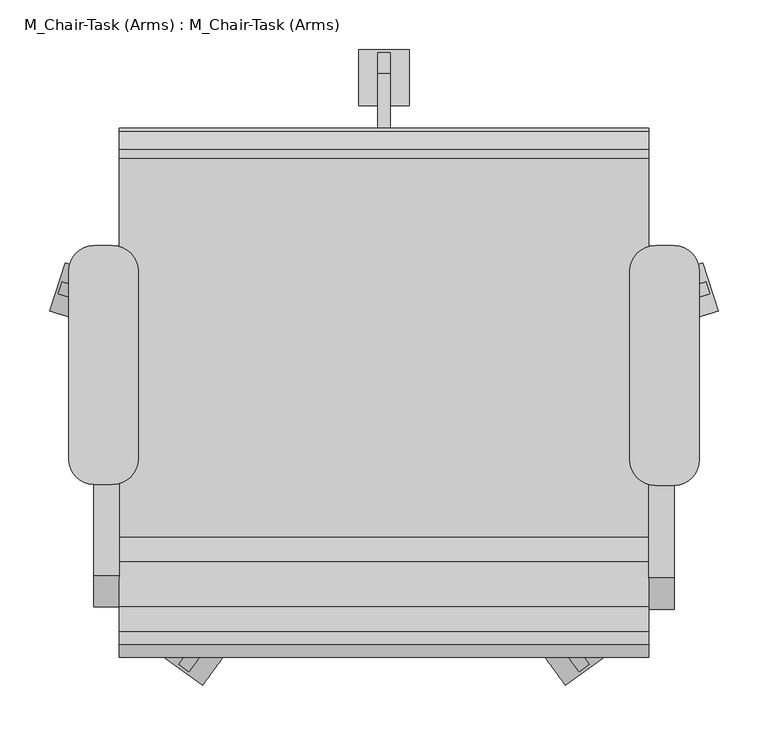
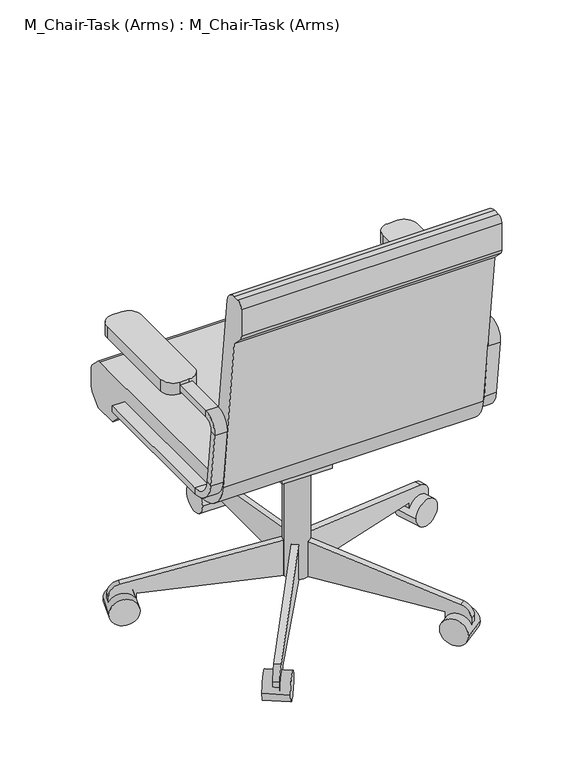
"""IFC4 building model written with IfcOpenShell, lengths in millimetres: furniture geometry, M_Chair-Task (Arms) : M_Chair-Task (Arms)."""

from ifc_helpers import new_model, si_unit, point, frame, frame_2d, origin, place, context, project, spatial, polyline, circle_curve, trimmed, segment, composite_curve, outline, extrude, source, transform, mapped, element, save
from ifc_brep_helpers import plane_surface, cylinder_surface, revolved_surface, advanced_brep


def m_chair_task_arms_m_chair_task_arms_fa5a08ef(model_context):
    return source(origin(), model_context, "Body", "SolidModel", [
        extrude(outline(composite_curve([segment(polyline([(433.0908197, -74.2028048), (414.0408197, -74.2028048)]), True, "CONTINUOUS"), segment(trimmed(circle_curve(frame_2d((414.0408197, -48.8028048)), 25.4), [point((414.0408197, -74.2028048))], [point((388.6408197, -48.8028048))], False, "CARTESIAN"), True, "CONTINUOUS"), segment(polyline([(388.6408197, -48.8028048), (388.6408197, 141.6319091)]), True, "CONTINUOUS"), segment(trimmed(circle_curve(frame_2d((414.0408197, 141.6319091)), 25.4), [point((388.6408197, 141.6319091))], [point((414.0408197, 167.0319091))], False, "CARTESIAN"), True, "CONTINUOUS"), segment(polyline([(414.0408197, 167.0319091), (433.0908197, 167.0319091)]), True, "CONTINUOUS"), segment(trimmed(circle_curve(frame_2d((433.0908197, 141.6319091)), 25.4), [point((433.0908197, 167.0319091))], [point((458.4908197, 141.6319091))], False, "CARTESIAN"), True, "CONTINUOUS"), segment(polyline([(458.4908197, 141.6319091), (458.4908197, -48.8028048)]), True, "CONTINUOUS"), segment(trimmed(circle_curve(frame_2d((433.0908197, -48.8028048)), 25.4), [point((458.4908197, -48.8028048))], [point((433.0908197, -74.2028048))], False, "CARTESIAN"), True, "CONTINUOUS")], self_intersect=False)), frame((0.0, 0.0, 596.9), z_axis=(0.0, 0.0, 1.0), x_axis=(1.0, 0.0, 0.0)), (0.0, 0.0, 1.0), 25.4),
        extrude(outline(composite_curve([segment(polyline([(-132.0591803, -73.1575984), (-151.1091803, -73.1575984)]), True, "CONTINUOUS"), segment(trimmed(circle_curve(frame_2d((-151.1091803, -47.7575984)), 25.4), [point((-151.1091803, -73.1575984))], [point((-176.5091803, -47.7575984))], False, "CARTESIAN"), True, "CONTINUOUS"), segment(polyline([(-176.5091803, -47.7575984), (-176.5091803, 141.6319091)]), True, "CONTINUOUS"), segment(trimmed(circle_curve(frame_2d((-151.1091803, 141.6319091)), 25.4), [point((-176.5091803, 141.6319091))], [point((-151.1091803, 167.0319091))], False, "CARTESIAN"), True, "CONTINUOUS"), segment(polyline([(-151.1091803, 167.0319091), (-132.0591803, 167.0319091)]), True, "CONTINUOUS"), segment(trimmed(circle_curve(frame_2d((-132.0591803, 141.6319091)), 25.4), [point((-132.0591803, 167.0319091))], [point((-106.6591803, 141.6319091))], False, "CARTESIAN"), True, "CONTINUOUS"), segment(polyline([(-106.6591803, 141.6319091), (-106.6591803, -47.7575984)]), True, "CONTINUOUS"), segment(trimmed(circle_curve(frame_2d((-132.0591803, -47.7575984)), 25.4), [point((-106.6591803, -47.7575984))], [point((-132.0591803, -73.1575984))], False, "CARTESIAN"), True, "CONTINUOUS")], self_intersect=False)), frame((0.0, 0.0, 596.9), z_axis=(0.0, 0.0, 1.0), x_axis=(1.0, 0.0, 0.0)), (0.0, 0.0, 1.0), 25.4),
        advanced_brep(
        [(-151.1091803, 167.0319091, 412.75), (-151.1091803, 167.0319091, 425.45), (-125.7091803, 167.0319091, 425.45), (-125.7091803, 167.0319091, 412.75), (-151.1091803, -126.2388651, 412.75), (-151.1091803, -126.2388651, 425.45), (-125.7091803, -126.2388651, 425.45), (-125.7091803, -126.2388651, 412.75), (-151.1091803, -170.3844094, 464.7064065), (-151.1091803, -182.9974221, 463.2225227), (-125.7091803, -170.3844094, 464.7064065), (-125.7091803, -182.9974221, 463.2225227), (-151.1091803, -196.7936301, 580.4902904), (-151.1091803, -184.1806174, 581.9741742), (-125.7091803, -184.1806174, 581.9741742), (-125.7091803, -196.7936301, 580.4902904), (-151.1091803, -165.2610984, 603.25), (-151.1091803, -165.2610984, 615.95), (-125.7091803, -165.2610984, 603.25), (-125.7091803, -165.2610984, 615.95), (-151.1091803, 18.9459016, 615.95), (-125.7091803, 18.9459016, 615.95), (-125.7091803, 18.9459016, 603.25), (-151.1091803, 18.9459016, 603.25)],
        [
            (0, 1),
            (1, 2),
            (2, 3),
            (3, 0),
            (0, 4),
            (4, 5),
            (5, 1),
            (5, 6),
            (6, 2),
            (6, 7),
            (7, 3),
            (7, 4),
            (8, 5, circle_curve(frame((-151.1091803, -126.2388651, 469.9), z_axis=(1.0, 0.0, 0.0), x_axis=(0.0, 0.0, -1.0)), 44.45)),
            (4, 9, circle_curve(frame((-151.1091803, -126.2388651, 469.9), z_axis=(-1.0, 0.0, 0.0), x_axis=(0.0, 0.0, -1.0)), 57.15)),
            (9, 8),
            (10, 6, circle_curve(frame((-125.7091803, -126.2388651, 469.9), z_axis=(1.0, 0.0, 0.0), x_axis=(0.0, 0.0, -1.0)), 44.45)),
            (8, 10),
            (11, 7, circle_curve(frame((-125.7091803, -126.2388651, 469.9), z_axis=(1.0, 0.0, 0.0), x_axis=(0.0, 0.0, -1.0)), 57.15)),
            (10, 11),
            (11, 9),
            (9, 12),
            (12, 13),
            (13, 8),
            (13, 14),
            (14, 10),
            (14, 15),
            (15, 11),
            (15, 12),
            (16, 13, circle_curve(frame((-151.1091803, -165.2610984, 584.2), z_axis=(1.0, 0.0, 0.0), x_axis=(0.0, -0.9931506043228768, -0.11684124756739202)), 19.05)),
            (12, 17, circle_curve(frame((-151.1091803, -165.2610984, 584.2), z_axis=(-1.0, 0.0, 0.0), x_axis=(0.0, -0.9931506043228768, -0.11684124756739202)), 31.75)),
            (17, 16),
            (18, 14, circle_curve(frame((-125.7091803, -165.2610984, 584.2), z_axis=(1.0, 0.0, 0.0), x_axis=(0.0, -0.9931506043228768, -0.11684124756739202)), 19.05)),
            (16, 18),
            (19, 15, circle_curve(frame((-125.7091803, -165.2610984, 584.2), z_axis=(1.0, 0.0, 0.0), x_axis=(0.0, -0.9931506043228768, -0.11684124756739202)), 31.75)),
            (18, 19),
            (19, 17),
            (20, 21),
            (21, 22),
            (22, 23),
            (23, 20),
            (17, 20),
            (23, 16),
            (22, 18),
            (21, 19),
        ],
        [
            plane_surface(frame((-152.608212, 167.0319091, 419.1), z_axis=(0.0, 1.0, 0.0), x_axis=(0.0, 0.0, -1.0))),
            plane_surface(frame((-151.1091803, 167.0319091, 412.75), z_axis=(-1.0, 0.0, 0.0), x_axis=(0.0, -1.0, 0.0))),
            plane_surface(frame((-151.1091803, 167.0319091, 425.45), z_axis=(0.0, 0.0, 1.0), x_axis=(0.0, -1.0, 0.0))),
            plane_surface(frame((-125.7091803, 167.0319091, 425.45), z_axis=(1.0, 0.0, 0.0), x_axis=(0.0, -1.0, 0.0))),
            plane_surface(frame((-125.7091803, 167.0319091, 412.75), z_axis=(0.0, 0.0, -1.0), x_axis=(0.0, -1.0, 0.0))),
            plane_surface(frame((-151.1091803, -126.2388651, 469.9), z_axis=(-1.0, 0.0, 0.0), x_axis=(0.0, 0.0, -1.0))),
            revolved_surface(polyline([(-151.1091803, -126.2388651, 425.45), (-125.7091803, -126.2388651, 425.45)]), (-138.4091803, -126.2388651, 469.9), (-1.0, 0.0, 0.0)),
            plane_surface(frame((-125.7091803, -126.2388651, 469.9), z_axis=(1.0, 0.0, 0.0), x_axis=(0.0, 0.0, -1.0))),
            cylinder_surface(frame((-138.4091803, -126.2388651, 469.9), z_axis=(-1.0, 0.0, 0.0), x_axis=(0.0, 0.0, -1.0)), 57.15),
            plane_surface(frame((-151.1091803, -182.9974221, 463.2225227), z_axis=(-1.0, 0.0, 0.0), x_axis=(0.0, -0.1168412475673856, 0.9931506043228776))),
            plane_surface(frame((-151.1091803, -170.3844094, 464.7064065), z_axis=(0.0, 0.9931506043228776, 0.1168412475673856), x_axis=(0.0, -0.1168412475673856, 0.9931506043228776))),
            plane_surface(frame((-125.7091803, -170.3844094, 464.7064065), z_axis=(1.0, 0.0, 0.0), x_axis=(0.0, -0.1168412475673856, 0.9931506043228776))),
            plane_surface(frame((-125.7091803, -182.9974221, 463.2225227), z_axis=(0.0, -0.9931506043228776, -0.1168412475673856), x_axis=(0.0, -0.1168412475673856, 0.9931506043228776))),
            plane_surface(frame((-151.1091803, -165.2610984, 584.2), z_axis=(-1.0, 0.0, 0.0), x_axis=(0.0, -0.9931506043228768, -0.11684124756739202))),
            revolved_surface(polyline([(-151.1091803, -184.1806174123508, 581.9741742338413), (-125.7091803, -184.1806174123508, 581.9741742338413)]), (-138.4091803, -165.2610984, 584.2), (-1.0, 0.0, 0.0)),
            plane_surface(frame((-125.7091803, -165.2610984, 584.2), z_axis=(1.0, 0.0, 0.0), x_axis=(0.0, -0.9931506043228768, -0.11684124756739202))),
            cylinder_surface(frame((-138.4091803, -165.2610984, 584.2), z_axis=(-1.0, 0.0, 0.0), x_axis=(0.0, -0.9931506043228768, -0.11684124756739202)), 31.75),
            plane_surface(frame((-152.608212, 18.9459016, 609.6), z_axis=(0.0, 1.0, 0.0), x_axis=(0.0, 0.0, 1.0))),
            plane_surface(frame((-151.1091803, -165.2610984, 615.95), z_axis=(-1.0, 0.0, 0.0), x_axis=(0.0, 1.0, 0.0))),
            plane_surface(frame((-151.1091803, -165.2610984, 603.25), z_axis=(0.0, 0.0, -1.0), x_axis=(0.0, 1.0, 0.0))),
            plane_surface(frame((-125.7091803, -165.2610984, 603.25), z_axis=(1.0, 0.0, 0.0), x_axis=(0.0, 1.0, 0.0))),
            plane_surface(frame((-125.7091803, -165.2610984, 615.95), z_axis=(0.0, 0.0, 1.0), x_axis=(0.0, 1.0, 0.0))),
        ],
        [
            (0, [[1, 2, 3, 4]]),
            (1, [[-1, 5, 6, 7]]),
            (2, [[-2, -7, 8, 9]]),
            (3, [[-3, -9, 10, 11]]),
            (4, [[-4, -11, 12, -5]]),
            (5, [[13, -6, 14, 15]]),
            (6, [[16, -8, -13, 17]]),
            (7, [[18, -10, -16, 19]]),
            (8, [[-14, -12, -18, 20]]),
            (9, [[-15, 21, 22, 23]]),
            (10, [[-17, -23, 24, 25]]),
            (11, [[-19, -25, 26, 27]]),
            (12, [[-20, -27, 28, -21]]),
            (13, [[29, -22, 30, 31]]),
            (14, [[32, -24, -29, 33]]),
            (15, [[34, -26, -32, 35]]),
            (16, [[-30, -28, -34, 36]]),
            (17, [[37, 38, 39, 40]]),
            (18, [[-31, 41, -40, 42]]),
            (19, [[-33, -42, -39, 43]]),
            (20, [[-35, -43, -38, 44]]),
            (21, [[-36, -44, -37, -41]]),
        ],
    ),
        advanced_brep(
        [(433.0908197, 167.0319091, 425.45), (433.0908197, 167.0319091, 412.75), (407.6908197, 167.0319091, 412.75), (407.6908197, 167.0319091, 425.45), (433.0908197, -128.329278, 425.45), (433.0908197, -128.329278, 412.75), (407.6908197, -128.329278, 412.75), (407.6908197, -128.329278, 425.45), (433.0908197, -185.0878351, 463.2225227), (433.0908197, -172.4748224, 464.7064065), (407.6908197, -185.0878351, 463.2225227), (407.6908197, -172.4748224, 464.7064065), (433.0908197, -186.2710303, 581.9741742), (433.0908197, -198.884043, 580.4902904), (407.6908197, -198.884043, 580.4902904), (407.6908197, -186.2710303, 581.9741742), (433.0908197, -167.3515113, 615.95), (433.0908197, -167.3515113, 603.25), (407.6908197, -167.3515113, 615.95), (407.6908197, -167.3515113, 603.25), (433.0908197, 18.9459016, 603.25), (407.6908197, 18.9459016, 603.25), (407.6908197, 18.9459016, 615.95), (433.0908197, 18.9459016, 615.95)],
        [
            (0, 1),
            (1, 2),
            (2, 3),
            (3, 0),
            (0, 4),
            (4, 5),
            (5, 1),
            (5, 6),
            (6, 2),
            (6, 7),
            (7, 3),
            (7, 4),
            (8, 5, circle_curve(frame((433.0908197, -128.329278, 469.9), z_axis=(1.0, 0.0, 0.0), x_axis=(0.0, 0.0, -1.0)), 57.15)),
            (4, 9, circle_curve(frame((433.0908197, -128.329278, 469.9), z_axis=(-1.0, 0.0, 0.0), x_axis=(0.0, 0.0, -1.0)), 44.45)),
            (9, 8),
            (10, 6, circle_curve(frame((407.6908197, -128.329278, 469.9), z_axis=(1.0, 0.0, 0.0), x_axis=(0.0, 0.0, -1.0)), 57.15)),
            (8, 10),
            (11, 7, circle_curve(frame((407.6908197, -128.329278, 469.9), z_axis=(1.0, 0.0, 0.0), x_axis=(0.0, 0.0, -1.0)), 44.45)),
            (10, 11),
            (11, 9),
            (9, 12),
            (12, 13),
            (13, 8),
            (13, 14),
            (14, 10),
            (14, 15),
            (15, 11),
            (15, 12),
            (16, 13, circle_curve(frame((433.0908197, -167.3515113, 584.2), z_axis=(1.0, 0.0, 0.0), x_axis=(0.0, -0.9931506043228767, -0.1168412475673929)), 31.75)),
            (12, 17, circle_curve(frame((433.0908197, -167.3515113, 584.2), z_axis=(-1.0, 0.0, 0.0), x_axis=(0.0, -0.9931506043228767, -0.1168412475673929)), 19.05)),
            (17, 16),
            (18, 14, circle_curve(frame((407.6908197, -167.3515113, 584.2), z_axis=(1.0, 0.0, 0.0), x_axis=(0.0, -0.9931506043228767, -0.1168412475673929)), 31.75)),
            (16, 18),
            (19, 15, circle_curve(frame((407.6908197, -167.3515113, 584.2), z_axis=(1.0, 0.0, 0.0), x_axis=(0.0, -0.9931506043228767, -0.1168412475673929)), 19.05)),
            (18, 19),
            (19, 17),
            (20, 21),
            (21, 22),
            (22, 23),
            (23, 20),
            (17, 20),
            (23, 16),
            (22, 18),
            (21, 19),
        ],
        [
            plane_surface(frame((406.191788, 167.0319091, 419.1), z_axis=(0.0, 1.0, 0.0), x_axis=(0.0, 0.0, -1.0))),
            plane_surface(frame((433.0908197, 167.0319091, 425.45), z_axis=(1.0, 0.0, 0.0), x_axis=(0.0, -1.0, 0.0))),
            plane_surface(frame((433.0908197, 167.0319091, 412.75), z_axis=(0.0, 0.0, -1.0), x_axis=(0.0, -1.0, 0.0))),
            plane_surface(frame((407.6908197, 167.0319091, 412.75), z_axis=(-1.0, 0.0, 0.0), x_axis=(0.0, -1.0, 0.0))),
            plane_surface(frame((407.6908197, 167.0319091, 425.45), z_axis=(0.0, 0.0, 1.0), x_axis=(0.0, -1.0, 0.0))),
            plane_surface(frame((433.0908197, -128.329278, 469.9), z_axis=(1.0, 0.0, 0.0), x_axis=(0.0, 0.0, -1.0))),
            cylinder_surface(frame((420.3908197, -128.329278, 469.9), z_axis=(-1.0, 0.0, 0.0), x_axis=(0.0, 0.0, -1.0)), 57.15),
            plane_surface(frame((407.6908197, -128.329278, 469.9), z_axis=(-1.0, 0.0, 0.0), x_axis=(0.0, 0.0, -1.0))),
            revolved_surface(polyline([(407.6908197, -128.329278, 425.45), (433.0908197, -128.329278, 425.45)]), (420.3908197, -128.329278, 469.9), (-1.0, 0.0, 0.0)),
            plane_surface(frame((433.0908197, -172.4748224, 464.7064065), z_axis=(1.0, 0.0, 0.0), x_axis=(0.0, -0.11684124756738626, 0.9931506043228775))),
            plane_surface(frame((433.0908197, -185.0878351, 463.2225227), z_axis=(0.0, -0.9931506043228775, -0.11684124756738655), x_axis=(0.0, -0.11684124756738655, 0.9931506043228775))),
            plane_surface(frame((407.6908197, -185.0878351, 463.2225227), z_axis=(-1.0, 0.0, 0.0), x_axis=(0.0, -0.11684124756738626, 0.9931506043228775))),
            plane_surface(frame((407.6908197, -172.4748224, 464.7064065), z_axis=(0.0, 0.9931506043228775, 0.11684124756738626), x_axis=(0.0, -0.11684124756738626, 0.9931506043228775))),
            plane_surface(frame((433.0908197, -167.3515113, 584.2), z_axis=(1.0, 0.0, 0.0), x_axis=(0.0, -0.9931506043228767, -0.1168412475673929))),
            cylinder_surface(frame((420.3908197, -167.3515113, 584.2), z_axis=(-1.0, 0.0, 0.0), x_axis=(0.0, -0.9931506043228767, -0.1168412475673929)), 31.75),
            plane_surface(frame((407.6908197, -167.3515113, 584.2), z_axis=(-1.0, 0.0, 0.0), x_axis=(0.0, -0.9931506043228767, -0.1168412475673929))),
            revolved_surface(polyline([(407.6908197, -186.2710303123508, 581.9741742338412), (433.0908197, -186.2710303123508, 581.9741742338412)]), (420.3908197, -167.3515113, 584.2), (-1.0, 0.0, 0.0)),
            plane_surface(frame((406.191788, 18.9459016, 609.6), z_axis=(0.0, 1.0, 0.0), x_axis=(0.0, 0.0, 1.0))),
            plane_surface(frame((433.0908197, -167.3515113, 603.25), z_axis=(1.0, 0.0, 0.0), x_axis=(0.0, 1.0, 0.0))),
            plane_surface(frame((433.0908197, -167.3515113, 615.95), z_axis=(0.0, 0.0, 1.0), x_axis=(0.0, 1.0, 0.0))),
            plane_surface(frame((407.6908197, -167.3515113, 615.95), z_axis=(-1.0, 0.0, 0.0), x_axis=(0.0, 1.0, 0.0))),
            plane_surface(frame((407.6908197, -167.3515113, 603.25), z_axis=(0.0, 0.0, -1.0), x_axis=(0.0, 1.0, 0.0))),
        ],
        [
            (0, [[1, 2, 3, 4]]),
            (1, [[-1, 5, 6, 7]]),
            (2, [[-2, -7, 8, 9]]),
            (3, [[-3, -9, 10, 11]]),
            (4, [[-4, -11, 12, -5]]),
            (5, [[13, -6, 14, 15]]),
            (6, [[16, -8, -13, 17]]),
            (7, [[18, -10, -16, 19]]),
            (8, [[-14, -12, -18, 20]]),
            (9, [[-15, 21, 22, 23]]),
            (10, [[-17, -23, 24, 25]]),
            (11, [[-19, -25, 26, 27]]),
            (12, [[-20, -27, 28, -21]]),
            (13, [[29, -22, 30, 31]]),
            (14, [[32, -24, -29, 33]]),
            (15, [[34, -26, -32, 35]]),
            (16, [[-30, -28, -34, 36]]),
            (17, [[37, 38, 39, 40]]),
            (18, [[-31, 41, -40, 42]]),
            (19, [[-33, -42, -39, 43]]),
            (20, [[-35, -43, -38, 44]]),
            (21, [[-36, -44, -37, -41]]),
        ],
    ),
        extrude(outline(composite_curve([segment(trimmed(circle_curve(frame_2d((140.9908197, 18.9459016)), 25.4), [point((115.5908197, 18.9459016))], [point((166.3908197, 18.9459016))], False, "CARTESIAN"), True, "CONTINUOUS"), segment(trimmed(circle_curve(frame_2d((140.9908197, 18.9459016)), 25.4), [point((166.3908197, 18.9459016))], [point((115.5908197, 18.9459016))], False, "CARTESIAN"), True, "CONTINUOUS")], self_intersect=False)), frame((0.0, 0.0, 53.5835944), z_axis=(0.0, 0.0, 1.0), x_axis=(1.0, 0.0, 0.0)), (0.0, 0.0, 1.0), 330.5914056),
        extrude(outline(composite_curve([segment(trimmed(circle_curve(frame_2d((0.0, -28.2002727)), 28.2002727), [point((0.0, -56.4005455))], [point((0.0, 0.0))], False, "CARTESIAN"), True, "CONTINUOUS"), segment(trimmed(circle_curve(frame_2d((0.0, -28.2002727)), 28.2002727), [point((0.0, 0.0))], [point((0.0, -56.4005455))], False, "CARTESIAN"), True, "CONTINUOUS")], self_intersect=False)), frame((477.6203484, 101.6163254, 28.1835944), z_axis=(-0.3090169943749423, 0.9510565162951553, 0.0), x_axis=(0.0, 0.0, 1.0)), (0.0, 0.0, 1.0), 50.8),
        extrude(outline(composite_curve([segment(polyline([(-25.4, 0.0), (0.0, 0.0), (0.0, -50.8), (-24.303053, -50.8)]), True, "CONTINUOUS"), segment(trimmed(circle_curve(frame_2d((-24.303053, -25.4)), 25.4), [point((-24.303053, -50.8))], [point((-49.3171699, -29.8106637))], False, "CARTESIAN"), True, "CONTINUOUS"), segment(polyline([(-49.3171699, -29.8106637), (-101.6, 266.7), (-101.6, 292.1), (-25.4, 292.1), (-25.4, 0.0)]), True, "CONTINUOUS")], self_intersect=False)), frame((420.756686, 103.1705568, 28.1835944), z_axis=(-0.3090169943749423, 0.9510565162951553, 0.0), x_axis=(0.0, 0.0, -1.0)), (0.0, 0.0, 1.0), 12.7),
        extrude(outline(composite_curve([segment(trimmed(circle_curve(frame_2d((0.0, -28.2002727)), 28.2002727), [point((0.0, -56.4005455))], [point((0.0, 0.0))], False, "CARTESIAN"), True, "CONTINUOUS"), segment(trimmed(circle_curve(frame_2d((0.0, -28.2002727)), 28.2002727), [point((0.0, 0.0))], [point((0.0, -56.4005455))], False, "CARTESIAN"), True, "CONTINUOUS")], self_intersect=False)), frame((323.63931, -275.6612394, 28.1835944), z_axis=(0.8090169943749499, 0.5877852522924699, 0.0), x_axis=(0.0, 0.0, 1.0)), (0.0, 0.0, 1.0), 50.8),
        extrude(outline(composite_curve([segment(polyline([(-25.4, 0.0), (0.0, 0.0), (0.0, -50.8), (-24.303053, -50.8)]), True, "CONTINUOUS"), segment(trimmed(circle_curve(frame_2d((-24.303053, -25.3999999)), 25.4), [point((-24.303053, -50.8))], [point((-49.3171699, -29.8106636))], False, "CARTESIAN"), True, "CONTINUOUS"), segment(polyline([(-49.3171699, -29.8106636), (-101.6, 266.7), (-101.6, 292.1), (-25.4, 292.1), (-25.4, 0.0)]), True, "CONTINUOUS")], self_intersect=False)), frame((307.545634, -221.1003988, 28.1835944), z_axis=(0.8090169943749499, 0.5877852522924699, 0.0), x_axis=(0.0, 0.0, -1.0)), (0.0, 0.0, 1.0), 12.7),
        extrude(outline(composite_curve([segment(trimmed(circle_curve(frame_2d((0.0, -28.2002727)), 28.2002727), [point((0.0, -56.4005455))], [point((0.0, 0.0))], False, "CARTESIAN"), True, "CONTINUOUS"), segment(trimmed(circle_curve(frame_2d((0.0, -28.2002727)), 28.2002727), [point((0.0, 0.0))], [point((0.0, -56.4005455))], False, "CARTESIAN"), True, "CONTINUOUS")], self_intersect=False)), frame((-41.6576707, -275.6612394, 28.1835944), z_axis=(-0.8090169943749458, 0.5877852522924754, 0.0), x_axis=(0.0, 0.0, -1.0)), (0.0, 0.0, 1.0), 50.8),
        extrude(outline(composite_curve([segment(polyline([(25.4, 0.0), (25.4, 292.1), (101.6, 292.1), (101.6, 266.7), (49.3171699, -29.8106637)]), True, "CONTINUOUS"), segment(trimmed(circle_curve(frame_2d((24.303053, -25.3999999)), 25.4), [point((49.3171699, -29.8106637))], [point((24.303053, -50.8))], False, "CARTESIAN"), True, "CONTINUOUS"), segment(polyline([(24.303053, -50.8), (0.0, -50.8), (0.0, 0.0), (25.4, 0.0)]), True, "CONTINUOUS")], self_intersect=False)), frame((-25.5639946, -221.1003988, 28.1835944), z_axis=(-0.8090169943749459, 0.5877852522924754, 0.0), x_axis=(0.0, 0.0, 1.0)), (0.0, 0.0, 1.0), 12.7),
        extrude(outline(composite_curve([segment(trimmed(circle_curve(frame_2d((0.0, -28.2002727)), 28.2002727), [point((0.0, -56.4005454))], [point((0.0, 0.0))], False, "CARTESIAN"), True, "CONTINUOUS"), segment(trimmed(circle_curve(frame_2d((0.0, -28.2002727)), 28.2002727), [point((0.0, 0.0))], [point((0.0, -56.4005454))], False, "CARTESIAN"), True, "CONTINUOUS")], self_intersect=False)), frame((-195.638709, 101.6163254, 28.1835944), z_axis=(0.3090169943749487, 0.9510565162951532, 0.0), x_axis=(0.0, 0.0, -1.0)), (0.0, 0.0, 1.0), 50.8),
        extrude(outline(composite_curve([segment(polyline([(25.4, 0.0), (25.4, 292.1000001), (101.6, 292.1000001), (101.6, 266.7), (49.3171699, -29.8106636)]), True, "CONTINUOUS"), segment(trimmed(circle_curve(frame_2d((24.303053, -25.4)), 25.4), [point((49.3171699, -29.8106636))], [point((24.303053, -50.8))], False, "CARTESIAN"), True, "CONTINUOUS"), segment(polyline([(24.303053, -50.8), (0.0, -50.8), (0.0, 0.0), (25.4, 0.0)]), True, "CONTINUOUS")], self_intersect=False)), frame((-138.7750467, 103.1705568, 28.1835944), z_axis=(0.3090169943749487, 0.9510565162951532, 0.0), x_axis=(0.0, 0.0, 1.0)), (0.0, 0.0, 1.0), 12.7),
        extrude(outline(composite_curve([segment(trimmed(circle_curve(frame_2d((336.4459016, 28.1835944)), 28.2002727), [point((308.2456289, 28.1835944))], [point((364.6461744, 28.1835944))], False, "CARTESIAN"), True, "CONTINUOUS"), segment(trimmed(circle_curve(frame_2d((336.4459016, 28.1835944)), 28.2002727), [point((364.6461744, 28.1835944))], [point((308.2456289, 28.1835944))], False, "CARTESIAN"), True, "CONTINUOUS")], self_intersect=False)), frame((115.5908197, 0.0, 0.0), z_axis=(1.0, 0.0, 0.0), x_axis=(0.0, 1.0, 0.0)), (0.0, 0.0, 1.0), 50.8),
        extrude(outline(composite_curve([segment(polyline([(311.0459016, 53.5835944), (18.9459016, 53.5835944), (18.9459016, 129.7835944), (44.3459016, 129.7835944), (340.8565654, 77.5007643)]), True, "CONTINUOUS"), segment(trimmed(circle_curve(frame_2d((336.4459016, 52.4866474)), 25.4), [point((340.8565654, 77.5007643))], [point((361.8459016, 52.4866474))], False, "CARTESIAN"), True, "CONTINUOUS"), segment(polyline([(361.8459016, 52.4866474), (361.8459016, 28.1835944), (311.0459016, 28.1835944), (311.0459016, 53.5835944)]), True, "CONTINUOUS")], self_intersect=False)), frame((134.6408197, 0.0, 0.0), z_axis=(1.0, 0.0, 0.0), x_axis=(0.0, 1.0, 0.0)), (0.0, 0.0, 1.0), 12.7),
        extrude(outline(polyline([(69.7459016, 383.7835944), (69.7459016, 371.0835944), (18.9459016, 283.0954134), (-19.1540984, 283.0954134), (-19.1540984, 383.7835944), (69.7459016, 383.7835944)])), frame((90.1908197, 0.0, 0.0), z_axis=(1.0, 0.0, 0.0), x_axis=(0.0, 1.0, 0.0)), (0.0, 0.0, 1.0), 101.6),
        extrude(outline(composite_curve([segment(polyline([(-126.2050455, 457.2), (255.0102301, 457.2)]), True, "CONTINUOUS"), segment(trimmed(circle_curve(frame_2d((255.0102301, 444.5)), 12.7), [point((255.0102301, 457.2))], [point((263.9604301, 453.510212))], False, "CARTESIAN"), True, "CONTINUOUS"), segment(polyline([(263.9604301, 453.510212), (281.8961016, 435.6939999)]), True, "CONTINUOUS"), segment(trimmed(circle_curve(frame_2d((272.9459016, 426.6837879)), 12.7), [point((281.8961016, 435.6939999))], [point((285.6459016, 426.6837879))], False, "CARTESIAN"), True, "CONTINUOUS"), segment(polyline([(285.6459016, 426.6837879), (285.6459016, 391.6405184)]), True, "CONTINUOUS"), segment(trimmed(circle_curve(frame_2d((260.2459016, 391.6405184)), 25.4), [point((285.6459016, 391.6405184))], [point((278.2663256, 373.7401184))], False, "CARTESIAN"), True, "CONTINUOUS"), segment(polyline([(278.2663256, 373.7401184), (260.2470284, 355.6), (209.4470284, 355.6), (181.0744602, 383.7835944), (-107.1089978, 383.7835944)]), True, "CONTINUOUS"), segment(trimmed(circle_curve(frame_2d((-107.1089978, 459.9835944)), 76.2), [point((-107.1089978, 383.7835944))], [point((-182.7870738, 451.0802913))], False, "CARTESIAN"), True, "CONTINUOUS"), segment(polyline([(-182.7870738, 451.0802913), (-222.3540984, 787.4), (-244.0343545, 809.0802561)]), True, "CONTINUOUS"), segment(trimmed(circle_curve(frame_2d((-235.0540984, 818.0605122)), 12.7), [point((-244.0343545, 809.0802561))], [point((-247.7540984, 818.0605122))], False, "CARTESIAN"), True, "CONTINUOUS"), segment(polyline([(-247.7540984, 818.0605122), (-247.7540984, 876.3)]), True, "CONTINUOUS"), segment(trimmed(circle_curve(frame_2d((-235.0540984, 876.3)), 12.7), [point((-247.7540984, 876.3))], [point((-235.0540984, 889.0))], False, "CARTESIAN"), True, "CONTINUOUS"), segment(polyline([(-235.0540984, 889.0), (-222.1789239, 889.0)]), True, "CONTINUOUS"), segment(trimmed(circle_curve(frame_2d((-222.1789239, 863.6)), 25.4), [point((-222.1789239, 889.0))], [point((-196.9528985, 866.5677677))], False, "CARTESIAN"), True, "CONTINUOUS"), segment(polyline([(-196.9528985, 866.5677677), (-151.4310708, 479.6322323)]), True, "CONTINUOUS"), segment(trimmed(circle_curve(frame_2d((-126.2050455, 482.6)), 25.4), [point((-151.4310708, 479.6322323))], [point((-126.2050455, 457.2))], True, "CARTESIAN"), True, "CONTINUOUS")], self_intersect=False)), frame((-125.7091803, 0.0, 0.0), z_axis=(1.0, 0.0, 0.0), x_axis=(0.0, 1.0, 0.0)), (0.0, 0.0, 1.0), 533.4),
    ])


if __name__ == "__main__":
    model = new_model("IFC4")
    model_context = context("Model", 3, world=origin())
    ifc_project = project(units=[si_unit("LENGTHUNIT", "METRE", prefix="MILLI")], contexts=[model_context])
    site = spatial("IfcSite", under=ifc_project)
    building = spatial("IfcBuilding", under=site)
    placement = place(None, origin())
    m_chair_task_arms_m_chair_task_arms_shape = m_chair_task_arms_m_chair_task_arms_fa5a08ef(model_context)
    element("IfcFurniture", 1, ObjectType="M_Chair-Task (Arms) : M_Chair-Task (Arms)", at=placement, inside=building, context=model_context, shape_type="MappedRepresentation", body=[
        mapped(m_chair_task_arms_m_chair_task_arms_shape, transform((0.0, 0.0, 0.0), x_axis=(1.0, 0.0, 0.0), y_axis=(0.0, 1.0, 0.0), z_axis=(0.0, 0.0, 1.0))),
    ])
    save(model, "model.ifc")

# Revit data of these elements
# Type "M_Chair-Task (Arms) : M_Chair-Task (Arms)"
#   Base Material = Plastic, Opaque Black
#   Caster Material = Plastic, Opaque Black
#   Seat/Back Material = Textile - Slate Blue
#   Default Elevation = 0
# Element 1 (IfcFurniture, "M_Chair-Task (Arms) : M_Chair-Task (Arms)")
#   Materials on its faces: "Plastic, Opaque Black", "Textile - Slate Blue"
# Materials
#   "Plastic, Opaque Black": class "Plastic", colour RGB 0 0 0, transparency 0.7, Description = "Plastic, generic, opaque black", Cost = 0
#   "Textile - Slate Blue": class "Fabric", colour RGB 98 102 118, transparency 0
